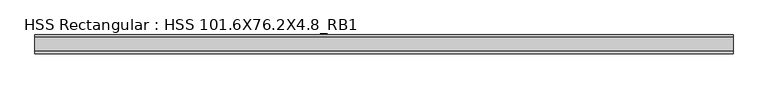
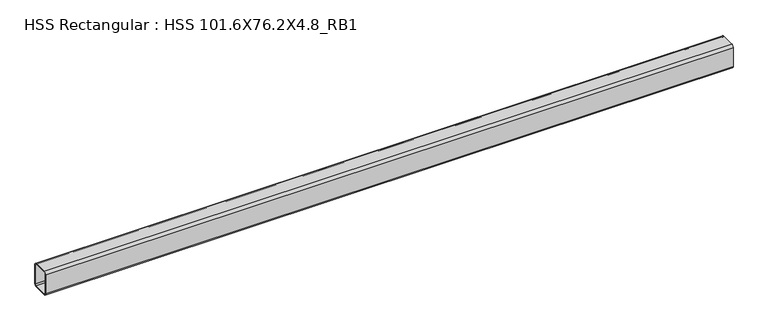
"""IFC4 building model written with IfcOpenShell, lengths in millimetres: beam geometry, HSS Rectangular : HSS 101.6X76.2X4.8_RB1."""

from ifc_helpers import new_model, si_unit, point, frame, frame_2d, origin, place, context, project, spatial, polyline, circle_curve, trimmed, segment, composite_curve, outline, extrude, source, transform, mapped, element, save


def hss_rectangular_hss_101_6x76_2x4_8_rb1_38707889(model_context):
    return source(origin(), model_context, "Body", "SweptSolid", [
        extrude(outline(composite_curve([segment(trimmed(circle_curve(frame_2d((-28.575, 41.275)), 9.525), [point((-38.1, 41.275))], [point((-28.575, 50.8))], False, "CARTESIAN"), True, "CONTINUOUS"), segment(polyline([(-28.575, 50.8), (28.575, 50.8)]), True, "CONTINUOUS"), segment(trimmed(circle_curve(frame_2d((28.575, 41.275)), 9.525), [point((28.575, 50.8))], [point((38.1, 41.275))], False, "CARTESIAN"), True, "CONTINUOUS"), segment(polyline([(38.1, 41.275), (38.1, -41.275)]), True, "CONTINUOUS"), segment(trimmed(circle_curve(frame_2d((28.575, -41.275)), 9.525), [point((38.1, -41.275))], [point((28.575, -50.8))], False, "CARTESIAN"), True, "CONTINUOUS"), segment(polyline([(28.575, -50.8), (-28.575, -50.8)]), True, "CONTINUOUS"), segment(trimmed(circle_curve(frame_2d((-28.575, -41.275)), 9.525), [point((-28.575, -50.8))], [point((-38.1, -41.275))], False, "CARTESIAN"), True, "CONTINUOUS"), segment(polyline([(-38.1, -41.275), (-38.1, 41.275)]), True, "CONTINUOUS")], self_intersect=False), holes=[composite_curve([segment(polyline([(28.575, 46.0375), (-28.575, 46.0375)]), True, "CONTINUOUS"), segment(trimmed(circle_curve(frame_2d((-28.575, 41.275)), 4.7625), [point((-28.575, 46.0375))], [point((-33.3375, 41.275))], True, "CARTESIAN"), True, "CONTINUOUS"), segment(polyline([(-33.3375, 41.275), (-33.3375, -41.275)]), True, "CONTINUOUS"), segment(trimmed(circle_curve(frame_2d((-28.575, -41.275)), 4.7625), [point((-33.3375, -41.275))], [point((-28.575, -46.0375))], True, "CARTESIAN"), True, "CONTINUOUS"), segment(polyline([(-28.575, -46.0375), (28.575, -46.0375)]), True, "CONTINUOUS"), segment(trimmed(circle_curve(frame_2d((28.575, -41.275)), 4.7625), [point((28.575, -46.0375))], [point((33.3375, -41.275))], True, "CARTESIAN"), True, "CONTINUOUS"), segment(polyline([(33.3375, -41.275), (33.3375, 41.275)]), True, "CONTINUOUS"), segment(trimmed(circle_curve(frame_2d((28.575, 41.275)), 4.7625), [point((33.3375, 41.275))], [point((28.575, 46.0375))], True, "CARTESIAN"), True, "CONTINUOUS")], self_intersect=False)]), frame((-1434.0933954, 0.0, 0.0), z_axis=(1.0, 0.0, 0.0), x_axis=(0.0, 1.0, 0.0)), (0.0, 0.0, 1.0), 2836.4367902),
    ])


if __name__ == "__main__":
    model = new_model("IFC4")
    model_context = context("Model", 3, world=origin())
    ifc_project = project(units=[si_unit("LENGTHUNIT", "METRE", prefix="MILLI")], contexts=[model_context])
    site = spatial("IfcSite", under=ifc_project)
    building = spatial("IfcBuilding", under=site)
    placement = place(None, origin())
    hss_rectangular_hss_101_6x76_2x4_8_rb1_shape = hss_rectangular_hss_101_6x76_2x4_8_rb1_38707889(model_context)
    element("IfcBeam", 1, ObjectType="HSS Rectangular : HSS 101.6X76.2X4.8_RB1", at=placement, inside=building, context=model_context, shape_type="MappedRepresentation", body=[
        mapped(hss_rectangular_hss_101_6x76_2x4_8_rb1_shape, transform((0.0, 0.0, 0.0), x_axis=(1.0, 0.0, 0.0), y_axis=(0.0, 1.0, 0.0), z_axis=(0.0, 0.0, 1.0))),
    ])
    save(model, "model.ifc")

# Revit data of these elements
# Type "HSS Rectangular : HSS 101.6X76.2X4.8_RB1"
#   Section Name Key = "HSS 4X3X3/16"
#   Assembly Code = "B10"
#   Width = 7.62 cm
#   Wall Nominal Thickness = 0.4763 cm
#   Wall Design Thickness = 0.442 cm
#   Torsional Moment of Inertia = 260.561 cm⁴
#   Torsional Modulus = 61.2876 cm³
#   Section Area = 14.4516 cm²
#   Plastic Modulus weak axis = 40.3122 cm³
#   Plastic Modulus strong axis = 49.1612 cm³
#   Perimeter = 0.881482 m²/m
#   Outer Fillet = 0.9525 cm
#   Nominal Weight = 12.1285 kgf/m
#   Moment of Inertia weak axis = 131.529 cm⁴
#   Moment of Inertia strong axis = 205.202 cm⁴
#   Inner Fillet = 0.4763 cm
#   Height = 10.16 cm
#   Elastic Modulus weak axis = 34.4128 cm³
#   Elastic Modulus strong axis = 40.476 cm³
#   Centroid Vertical = 5.08 cm
#   Centroid Horizontal = 3.81 cm
#   Length [instance default] = 1524 mm
#   Structural Material [instance default] = Steel ASTM A500, Grade B, Rectangular and Square
#   Principal Axes Angle = 0
# Element 1 (IfcBeam, "HSS Rectangular : HSS 101.6X76.2X4.8_RB1")
#   Structural Material = Steel ASTM A992
#   Materials on its faces: "Steel ASTM A992"
# Materials
#   "Steel ASTM A500, Grade B, Rectangular and Square": class "Metal", colour RGB 199 199 199, transparency 0, Description = "Carbon steel", Cost = 0
#   "Steel ASTM A992": class "Metal", colour RGB 199 199 199, transparency 0, Description = "Structural steel 50ksi", Cost = 0
